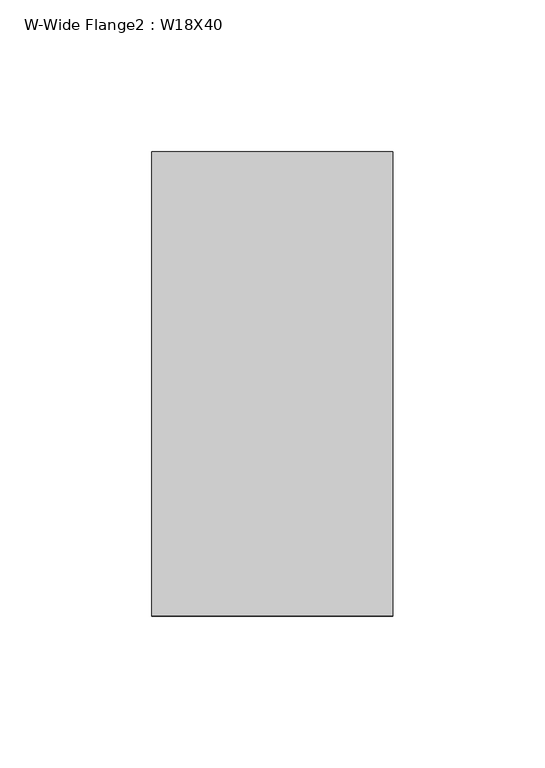
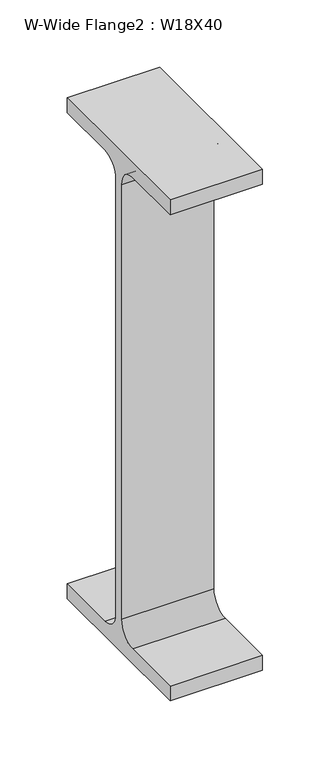
"""IFC4 building model written with IfcOpenShell, lengths in millimetres: beam geometry, W-Wide Flange2 : W18X40."""

from ifc_helpers import new_model, si_unit, point, frame, frame_2d, origin, place, context, project, spatial, polyline, circle_curve, trimmed, segment, composite_curve, outline, extrude, source, transform, mapped, element, save


def w_wide_flange2_w18x40_b68d0cc3(model_context):
    return source(origin(), model_context, "Body", "SweptSolid", [
        extrude(outline(composite_curve([segment(polyline([(76.454, -213.995), (76.454, -227.33), (-76.454, -227.33), (-76.454, -213.995), (-20.828, -213.995)]), True, "CONTINUOUS"), segment(trimmed(circle_curve(frame_2d((-20.828, -197.1675)), 16.8275), [point((-20.828, -213.995))], [point((-4.0005, -197.1675))], True, "CARTESIAN"), True, "CONTINUOUS"), segment(polyline([(-4.0005, -197.1675), (-4.0005, 197.1675)]), True, "CONTINUOUS"), segment(trimmed(circle_curve(frame_2d((-20.828, 197.1675)), 16.8275), [point((-4.0005, 197.1675))], [point((-20.828, 213.995))], True, "CARTESIAN"), True, "CONTINUOUS"), segment(polyline([(-20.828, 213.995), (-76.454, 213.995), (-76.454, 227.33), (76.454, 227.33), (76.454, 213.995), (20.828, 213.995)]), True, "CONTINUOUS"), segment(trimmed(circle_curve(frame_2d((20.828, 197.1675)), 16.8275), [point((20.828, 213.995))], [point((4.0005, 197.1675))], True, "CARTESIAN"), True, "CONTINUOUS"), segment(polyline([(4.0005, 197.1675), (4.0005, -197.1675)]), True, "CONTINUOUS"), segment(trimmed(circle_curve(frame_2d((20.828, -197.1675)), 16.8275), [point((4.0005, -197.1675))], [point((20.828, -213.995))], True, "CARTESIAN"), True, "CONTINUOUS"), segment(polyline([(20.828, -213.995), (76.454, -213.995)]), True, "CONTINUOUS")], self_intersect=False)), frame((-68.2625, 0.0, 0.0), z_axis=(1.0, 0.0, 0.0), x_axis=(0.0, 1.0, 0.0)), (0.0, 0.0, 1.0), 79.375),
    ])


if __name__ == "__main__":
    model = new_model("IFC4")
    model_context = context("Model", 3, world=origin())
    ifc_project = project(units=[si_unit("LENGTHUNIT", "METRE", prefix="MILLI")], contexts=[model_context])
    site = spatial("IfcSite", under=ifc_project)
    building = spatial("IfcBuilding", under=site)
    placement = place(None, origin())
    w_wide_flange2_w18x40_shape = w_wide_flange2_w18x40_b68d0cc3(model_context)
    element("IfcBeam", 1, ObjectType="W-Wide Flange2 : W18X40", at=placement, inside=building, context=model_context, shape_type="MappedRepresentation", body=[
        mapped(w_wide_flange2_w18x40_shape, transform((0.0, 0.0, 0.0), x_axis=(1.0, 0.0, 0.0), y_axis=(0.0, 1.0, 0.0), z_axis=(0.0, 0.0, 1.0))),
    ])
    save(model, "model.ifc")

# Revit data of these elements
# Type "W-Wide Flange2 : W18X40"
#   Assembly Code = "B10"
#   W = 40
#   Length [instance default] = 5' - 0"
#   bf = 0' - 6.02"
#   d = 1' - 5.9"
#   k = 0' - 1 3/16"
#   k2 = 0' - 0.6625"
#   tf = 0' - 0.525"
#   tw = 0' - 0.315"
#   A = 0.0819444 SF
#   Structural Material [instance default] = Steel ASTM A992
# Element 1 (IfcBeam, "W-Wide Flange2 : W18X40")
#   Materials on its faces: "Steel ASTM A992"
# Materials
#   "Steel ASTM A992": class "Metal", colour RGB 199 199 199, transparency 0, Description = "Structural steel 50ksi", Cost = 0
